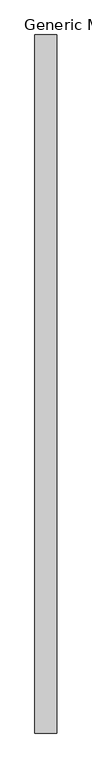
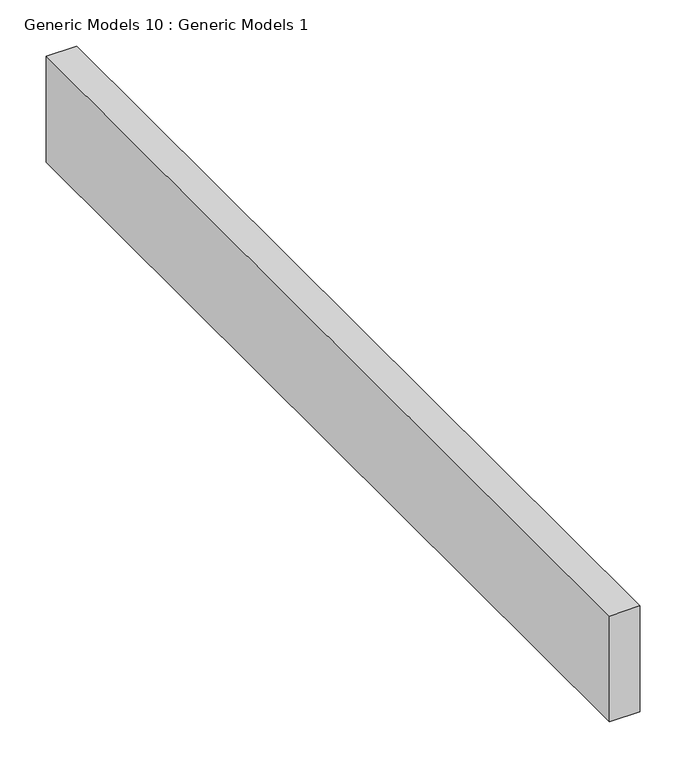
"""IFC4 building model written with IfcOpenShell, lengths in millimetres: proxy geometry, Generic Models 10 : Generic Models 1."""

import ifcopenshell
import ifcopenshell.guid

model = None  # the IFC model being written
_history = None  # IfcOwnerHistory: only IFC2X3 demands one
_inside = {}  # id of a spatial element -> (the spatial element, [elements in it])
_under = {}  # id of a project, library or spatial element -> (it, [spatial elements below it])
_declared = {}  # id of a project -> (the project, [libraries it declares])
_typed = {}  # id of a type object -> (the type object, [elements of that type])
_made_of = {}  # id of a material, layer set ... -> (it, [elements and type objects made of it])


def new_model(schema):
    """Start an empty IFC model of exactly this schema.

    Asked for "IFC4X3", IfcOpenShell would pick the latest addendum, in which some entities
    have other attributes; the version numbers below select the first issue.
    IFC2X3 requires an IfcOwnerHistory on every rooted entity: one is made here for all.
    """
    global model, _history
    if schema == "IFC4X3":
        model = ifcopenshell.file(schema_version=(4, 3, 0, 0))
    else:
        model = ifcopenshell.file(schema=schema)
    _inside.clear()
    _under.clear()
    _declared.clear()
    _typed.clear()
    _made_of.clear()
    _history = None
    if model.schema == "IFC2X3":
        org = make("IfcOrganization", Name="unknown")
        user = make(
            "IfcPersonAndOrganization",
            ThePerson=make("IfcPerson", FamilyName="unknown"),
            TheOrganization=org,
        )
        app = make(
            "IfcApplication",
            ApplicationDeveloper=org,
            Version="unknown",
            ApplicationFullName="unknown",
            ApplicationIdentifier="unknown",
        )
        _history = make(
            "IfcOwnerHistory",
            OwningUser=user,
            OwningApplication=app,
            ChangeAction="ADDED",
            CreationDate=0,
        )
    return model


def make(cls, **values):
    """One entity of the class cls with the attributes given. An attribute that is None is left unset."""
    return model.create_entity(
        cls, **{name: value for name, value in values.items() if value is not None}
    )


def rooted(cls, **values):
    """An entity with a GlobalId (a new one), such as an element, a storey or a relation."""
    return make(cls, GlobalId=ifcopenshell.guid.new(), OwnerHistory=_history, **values)


def si_unit(unit_type, name, prefix=None):
    """IfcSIUnit, for example si_unit("LENGTHUNIT", "METRE", prefix="MILLI")."""
    return make("IfcSIUnit", UnitType=unit_type, Prefix=prefix, Name=name)


def assignment(units):
    """IfcUnitAssignment: the units of a project."""
    return None if units is None else make("IfcUnitAssignment", Units=units)


def point(xyz):
    """IfcCartesianPoint."""
    return None if xyz is None else make("IfcCartesianPoint", Coordinates=xyz)


def direction(xyz):
    """IfcDirection."""
    return None if xyz is None else make("IfcDirection", DirectionRatios=xyz)


def frame(location, z_axis=None, x_axis=None):
    """IfcAxis2Placement3D, a coordinate frame: its origin and axes. An axis left out is left unset."""
    return make(
        "IfcAxis2Placement3D",
        Location=point(location),
        Axis=direction(z_axis),
        RefDirection=direction(x_axis),
    )


def origin():
    """The frame at (0, 0, 0) with its axes left unset."""
    return frame((0.0, 0.0, 0.0))


def place(relative_to, where):
    """IfcLocalPlacement: puts the frame where relative to a parent placement (None: the world)."""
    return make(
        "IfcLocalPlacement", PlacementRelTo=relative_to, RelativePlacement=where
    )


def context(
    kind, dimensions, precision=None, world=None, true_north=None, identifier=None
):
    """IfcGeometricRepresentationContext, for example the 3D "Model" context."""
    return make(
        "IfcGeometricRepresentationContext",
        ContextIdentifier=identifier,
        ContextType=kind,
        CoordinateSpaceDimension=dimensions,
        Precision=precision,
        WorldCoordinateSystem=world,
        TrueNorth=true_north,
    )


def project(units=None, contexts=None):
    """IfcProject with its units and contexts."""
    return rooted(
        "IfcProject",
        Name="project",
        RepresentationContexts=contexts,
        UnitsInContext=assignment(units),
    )


def spatial(cls, under=None, at=None, **own):
    """A site, building, storey or space (cls), placed at a placement, below another one or the project."""
    s = rooted(cls, ObjectPlacement=at, **own)
    if under is not None:
        _under.setdefault(under.id(), (under, []))[1].append(s)
    return s


def polyline(points):
    """IfcPolyline through the points."""
    return make("IfcPolyline", Points=[point(p) for p in points])


def outline(outer, holes=None, kind="AREA"):
    """IfcArbitraryClosedProfileDef: a profile drawn as a closed curve; with holes, ...WithVoids."""
    if holes is None:
        return make("IfcArbitraryClosedProfileDef", ProfileType=kind, OuterCurve=outer)
    return make(
        "IfcArbitraryProfileDefWithVoids",
        ProfileType=kind,
        OuterCurve=outer,
        InnerCurves=holes,
    )


def extrude(swept, where, along, depth):
    """IfcExtrudedAreaSolid: the profile swept, set in the frame where, extruded along a direction by depth."""
    return make(
        "IfcExtrudedAreaSolid",
        SweptArea=swept,
        Position=where,
        ExtrudedDirection=direction(along),
        Depth=depth,
    )


def shape(context_of_items, identifier, shape_type, items):
    """IfcShapeRepresentation: the items that make up one representation, for example the "Body"."""
    return make(
        "IfcShapeRepresentation",
        ContextOfItems=context_of_items,
        RepresentationIdentifier=identifier,
        RepresentationType=shape_type,
        Items=items,
    )


def source(mapping_origin, context_of_items, identifier, shape_type, items):
    """IfcRepresentationMap: a shape defined once, which mapped items show again and again."""
    return make(
        "IfcRepresentationMap",
        MappingOrigin=mapping_origin,
        MappedRepresentation=shape(context_of_items, identifier, shape_type, items),
    )


def transform(
    local_origin,
    x_axis=None,
    y_axis=None,
    z_axis=None,
    scale=None,
    scale2=None,
    scale3=None,
    uniform=True,
):
    """IfcCartesianTransformationOperator3D, or its non-uniform kind. x_axis, y_axis, z_axis: its Axis1, 2, 3."""
    if uniform:
        return make(
            "IfcCartesianTransformationOperator3D",
            Axis1=direction(x_axis),
            Axis2=direction(y_axis),
            LocalOrigin=point(local_origin),
            Scale=scale,
            Axis3=direction(z_axis),
        )
    return make(
        "IfcCartesianTransformationOperator3DnonUniform",
        Axis1=direction(x_axis),
        Axis2=direction(y_axis),
        LocalOrigin=point(local_origin),
        Scale=scale,
        Axis3=direction(z_axis),
        Scale2=scale2,
        Scale3=scale3,
    )


def mapped(mapping_source, mapping_target):
    """IfcMappedItem: shows the shape of a source again, moved by a transform."""
    return make(
        "IfcMappedItem", MappingSource=mapping_source, MappingTarget=mapping_target
    )


def made_of(thing, what):
    """Note that an element or type object is made of a material, layer set ...; save() writes the relation."""
    if what is not None:
        _made_of.setdefault(what.id(), (what, []))[1].append(thing)
    return thing


def element(
    cls,
    number,
    at=None,
    inside=None,
    cuts=None,
    type_object=None,
    material=None,
    context=None,
    identifier="Body",
    shape_type=None,
    held_by="IfcProductDefinitionShape",
    body=None,
    shapes=None,
    **own,
):
    """One element of the class cls, such as IfcWall. Its Tag is "e" and its number.

    at: its placement. inside: the storey or other place that contains it. cuts: it is an
    opening in that element (IfcRelVoidsElement). A single representation is given by context,
    identifier, shape_type and body (its items); several are given by shapes. held_by: the class
    of the entity that holds the representations. save() writes the other relations.
    """
    e = rooted(cls, Tag="e%d" % number, ObjectPlacement=at, **own)
    if body is not None:
        shapes = [shape(context, identifier, shape_type, body)]
    if shapes is not None:
        e.Representation = make(held_by, Representations=shapes)
    if inside is not None:
        _inside.setdefault(inside.id(), (inside, []))[1].append(e)
    if cuts is not None:
        rooted(
            "IfcRelVoidsElement", RelatingBuildingElement=cuts, RelatedOpeningElement=e
        )
    if type_object is not None:
        _typed.setdefault(type_object.id(), (type_object, []))[1].append(e)
    return made_of(e, material)


def aggregate(whole, parts):
    """IfcRelAggregates: a whole, such as a stair, and the parts it consists of."""
    return rooted("IfcRelAggregates", RelatingObject=whole, RelatedObjects=parts)


def save(model, path):
    """Write the relations noted so far, then the file.

    IfcRelAggregates (storeys below a building ...), IfcRelContainedInSpatialStructure (elements
    in a storey), IfcRelDefinesByType, IfcRelAssociatesMaterial and IfcRelDeclares: one each for
    every whole, place, type object, material and project.
    """
    for whole, parts in _under.values():
        aggregate(whole, parts)
    for where, things in _inside.values():
        rooted(
            "IfcRelContainedInSpatialStructure",
            RelatedElements=things,
            RelatingStructure=where,
        )
    for kind, things in _typed.values():
        rooted("IfcRelDefinesByType", RelatedObjects=things, RelatingType=kind)
    for what, things in _made_of.values():
        rooted("IfcRelAssociatesMaterial", RelatedObjects=things, RelatingMaterial=what)
    for by, libraries in _declared.values():
        rooted("IfcRelDeclares", RelatingContext=by, RelatedDefinitions=libraries)
    model.write(path)


def generic_models_10_generic_models_1_ea081297(model_context):
    return source(origin(), model_context, "Body", "SweptSolid", [
        extrude(outline(polyline([(49758.6, 0.0), (49720.5, 0.0), (49720.5, 1219.2), (49758.6, 1219.2), (49758.6, 0.0)])), frame((0.0, 0.0, 5507.83125), z_axis=(0.0, 0.0, 1.0), x_axis=(1.0, 0.0, 0.0)), (0.0, 0.0, 1.0), 139.7),
    ])


if __name__ == "__main__":
    model = new_model("IFC4")
    model_context = context("Model", 3, world=origin())
    ifc_project = project(units=[si_unit("LENGTHUNIT", "METRE", prefix="MILLI")], contexts=[model_context])
    site = spatial("IfcSite", under=ifc_project)
    building = spatial("IfcBuilding", under=site)
    placement = place(None, origin())
    generic_models_10_generic_models_1_shape = generic_models_10_generic_models_1_ea081297(model_context)
    element("IfcBuildingElementProxy", 1, Name="Generic Models 10 : Generic Models 1", ObjectType="Generic Models 10 : Generic Models 1", at=placement, inside=building, context=model_context, shape_type="MappedRepresentation", body=[
        mapped(generic_models_10_generic_models_1_shape, transform((0.0, 0.0, 0.0), x_axis=(1.0, 0.0, 0.0), y_axis=(0.0, 1.0, 0.0), z_axis=(0.0, 0.0, 1.0))),
    ])
    save(model, "model.ifc")

# Revit data of these elements
# Element 1 (IfcBuildingElementProxy, "Generic Models 10 : Generic Models 1")
#   Materials on its faces: "2X BLOCKING - LOCATED AT GRAB BARS, WALL HUNG CABINETS, ETC.)"
# Materials
#   "2X BLOCKING - LOCATED AT GRAB BARS, WALL HUNG CABINETS, ETC.)": class "Wood", colour RGB 234 198 147, transparency 0, Description = "Pinus Echinata", Cost = 0
